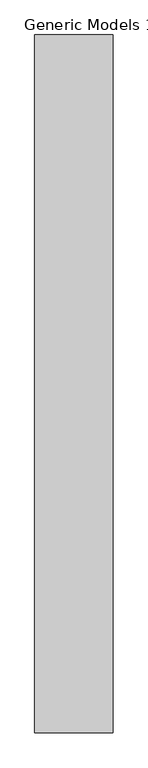
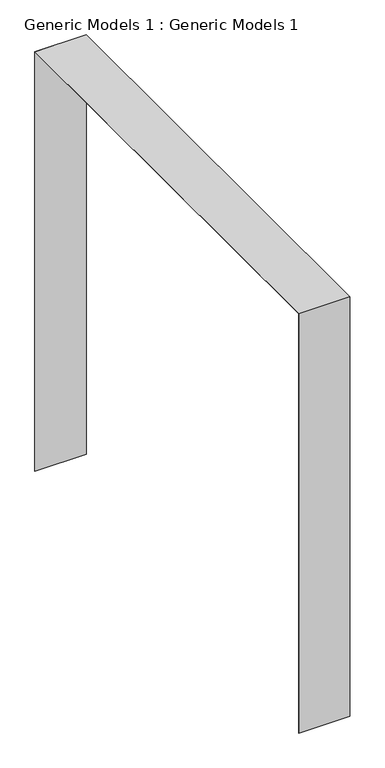
"""IFC4 building model written with IfcOpenShell, lengths in millimetres: proxy geometry, Generic Models 1 : Generic Models 1."""

from ifc_helpers import new_model, si_unit, frame, origin, place, context, project, spatial, polyline, outline, extrude, source, transform, mapped, element, save


def generic_models_1_generic_models_1_6dc33216(model_context):
    return source(origin(), model_context, "Body", "SweptSolid", [
        extrude(outline(polyline([(26552.7208589, 1749.9720055), (26551.7208589, 1749.9720055), (26551.7208589, 6598.9720055), (21553.7208589, 6598.9720055), (21553.7208589, 1749.9720055), (21552.7208589, 1749.9720055), (21552.7208589, 6599.9720055), (26552.7208589, 6599.9720055), (26552.7208589, 1749.9720055)])), frame((-935.0, 0.0, 0.0), z_axis=(1.0, 0.0, 0.0), x_axis=(0.0, 1.0, 0.0)), (0.0, 0.0, 1.0), 560.0),
    ])


if __name__ == "__main__":
    model = new_model("IFC4")
    model_context = context("Model", 3, world=origin())
    ifc_project = project(units=[si_unit("LENGTHUNIT", "METRE", prefix="MILLI")], contexts=[model_context])
    site = spatial("IfcSite", under=ifc_project)
    building = spatial("IfcBuilding", under=site)
    placement = place(None, origin())
    generic_models_1_generic_models_1_shape = generic_models_1_generic_models_1_6dc33216(model_context)
    element("IfcBuildingElementProxy", 1, Name="Generic Models 1 : Generic Models 1", ObjectType="Generic Models 1 : Generic Models 1", at=placement, inside=building, context=model_context, shape_type="MappedRepresentation", body=[
        mapped(generic_models_1_generic_models_1_shape, transform((0.0, 0.0, 0.0), x_axis=(1.0, 0.0, 0.0), y_axis=(0.0, 1.0, 0.0), z_axis=(0.0, 0.0, 1.0))),
    ])
    save(model, "model.ifc")
